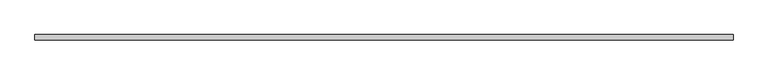
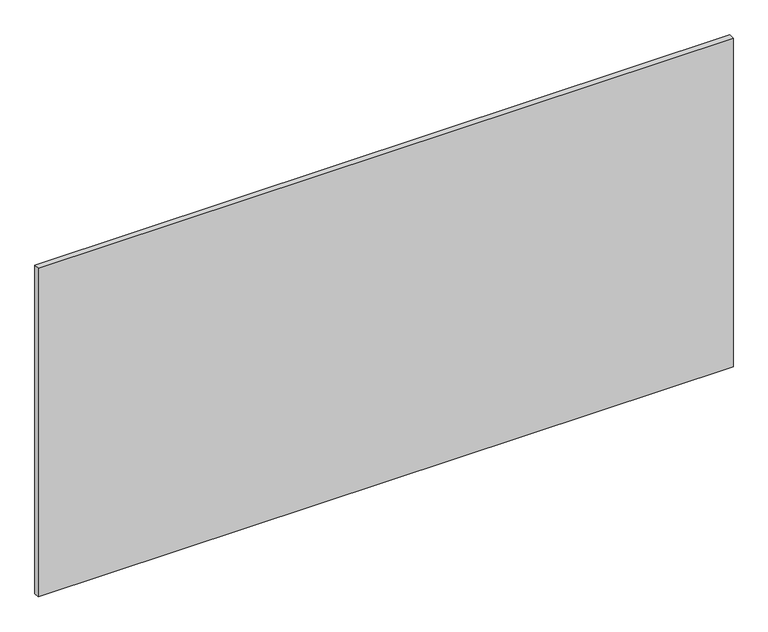
"""IFC4 building model written with IfcOpenShell, lengths in millimetres: proxy geometry, Inner panel:Inner panel:1:Inner panel:1 : Inner panel:Inner panel:300324:300043:Inner panel:1:Inner panel:1 : Inner panel:Inner panel:300324:300043 : Inner panel:Inner panel:1:Inner panel:1 : Inner panel:Inner panel:300324:300043:19 : Inner panel:Inner panel:1:Inner panel:1 : Inner panel:Inner panel:300324:300043:Inner panel:1:Inner panel:1 : Inner panel:Inner panel:300324:300043 : Inner panel:Inner panel:1:Inner panel:1 : Inner panel:Inner panel:300324:300043:300031."""

from ifc_helpers import new_model, si_unit, frame, origin, place, context, project, spatial, polyline, outline, extrude, source, transform, mapped, element, save


def generic_models_e9f893d6(model_context):
    return source(origin(), model_context, "Body", "SweptSolid", [
        extrude(outline(polyline([(594957.2867242, -568186.6413841), (597395.6867242, -568186.6413841), (597395.6867242, -568205.6913841), (594957.2867242, -568205.6913841), (594957.2867242, -568186.6413841)])), frame((0.0, 0.0, 3721.1), z_axis=(0.0, 0.0, 1.0), x_axis=(1.0, 0.0, 0.0)), (0.0, 0.0, 1.0), 1219.2),
    ])


if __name__ == "__main__":
    model = new_model("IFC4")
    model_context = context("Model", 3, world=origin())
    ifc_project = project(units=[si_unit("LENGTHUNIT", "METRE", prefix="MILLI")], contexts=[model_context])
    site = spatial("IfcSite", under=ifc_project)
    building = spatial("IfcBuilding", under=site)
    placement = place(None, origin())
    generic_models_shape = generic_models_e9f893d6(model_context)
    element("IfcBuildingElementProxy", 1, Name="Inner panel:Inner panel:1:Inner panel:1 : Inner panel:Inner panel:300324:300043:Inner panel:1:Inner panel:1 : Inner panel:Inner panel:300324:300043 : Inner panel:Inner panel:1:Inner panel:1 : Inner panel:Inner panel:300324:300043:19 : Inner panel:Inner panel:1:Inner panel:1 : Inner panel:Inner panel:300324:300043:Inner panel:1:Inner panel:1 : Inner panel:Inner panel:300324:300043 : Inner panel:Inner panel:1:Inner panel:1 : Inner panel:Inner panel:300324:300043:300031", ObjectType="Inner panel:Inner panel:1:Inner panel:1 : Inner panel:Inner panel:300324:300043:Inner panel:1:Inner panel:1 : Inner panel:Inner panel:300324:300043 : Inner panel:Inner panel:1:Inner panel:1 : Inner panel:Inner panel:300324:300043:19 : Inner panel:Inner panel:1:Inner panel:1 : Inner panel:Inner panel:300324:300043:Inner panel:1:Inner panel:1 : Inner panel:Inner panel:300324:300043 : Inner panel:Inner panel:1:Inner panel:1 : Inner panel:Inner panel:300324:300043:300031", at=placement, inside=building, context=model_context, shape_type="MappedRepresentation", body=[
        mapped(generic_models_shape, transform((0.0, 0.0, 0.0), x_axis=(1.0, 0.0, 0.0), y_axis=(0.0, 1.0, 0.0), z_axis=(0.0, 0.0, 1.0))),
    ])
    save(model, "model.ifc")

# Revit data of these elements
# Type "Inner panel:Inner panel:1:Inner panel:1 : Inner panel:Inner panel:300324:300043:Inner panel:1:Inner panel:1 : Inner panel:Inner panel:300324:300043 : Inner panel:Inner panel:1:Inner panel:1 : Inner panel:Inner panel:300324:300043:19 : Inner panel:Inner panel:1:Inner panel:1 : Inner panel:Inner panel:300324:300043:Inner panel:1:Inner panel:1 : Inner panel:Inner panel:300324:300043 : Inner panel:Inner panel:1:Inner panel:1 : Inner panel:Inner panel:300324:300043:300031"
#   NameOverride = "Inner panel:Inner panel:1:Inner panel:1 : Inner panel:Inner panel:300324:300043:Inner panel:1:Inner panel:1 : Inner panel:Inner panel:300324:300043 : Inner panel:Inner panel:1:Inner panel:1 : Inner panel:Inner panel:300324:300043:300031"
#   ObjectTypeOverride = "Inner panel:1:Inner panel:1 : Inner panel:Inner panel:300324:300043 : Inner panel:Inner panel:1:Inner panel:1 : Inner panel:Inner panel:300324:300043"
#   Reference = "Inner panel"
#   Tag = "300031"
# Element 1 (IfcBuildingElementProxy, "Inner panel:Inner panel:1:Inner panel:1 : Inner panel:Inner panel:300324:300043:Inner panel:1:Inner panel:1 : Inner panel:Inner panel:300324:300043 : Inner panel:Inner panel:1:Inner panel:1 : Inner panel:Inner panel:300324:300043:19 : Inner panel:Inner panel:1:Inner panel:1 : Inner panel:Inner panel:300324:300043:Inner panel:1:Inner panel:1 : Inner panel:Inner panel:300324:300043 : Inner panel:Inner panel:1:Inner panel:1 : Inner panel:Inner panel:300324:300043:300031")
#   Materials on its faces: "¾” (CLASS A) FIRE RETARDANT PLYWOOD ...OR… IF 1/4\" GYP. BD UNDER PLYWOOD, FLAME SPREAD TO BE CLASS C -  (FINISH: GRADE B - PREFINISHED STAINED/SEALED) - 1/4\" GAP BTWN PANELS (FASTENERS T.B.D.)"
# Materials
#   "¾” (CLASS A) FIRE RETARDANT PLYWOOD ...OR… IF 1/4\" GYP. BD UNDER PLYWOOD, FLAME SPREAD TO BE CLASS C -  (FINISH: GRADE B - PREFINISHED STAINED/SEALED) - 1/4\" GAP BTWN PANELS (FASTENERS T.B.D.)": class "Wood", colour RGB 149 120 74, transparency 0, Description = "Plywood, sheathing grade", Cost = 0
